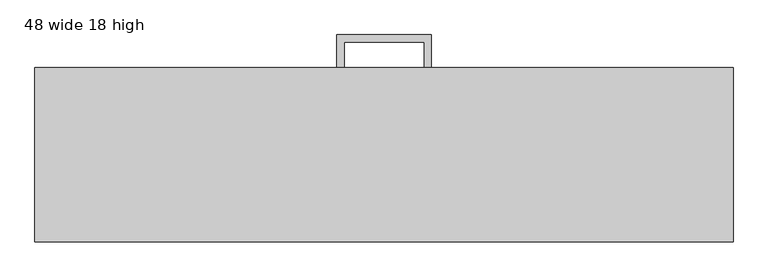
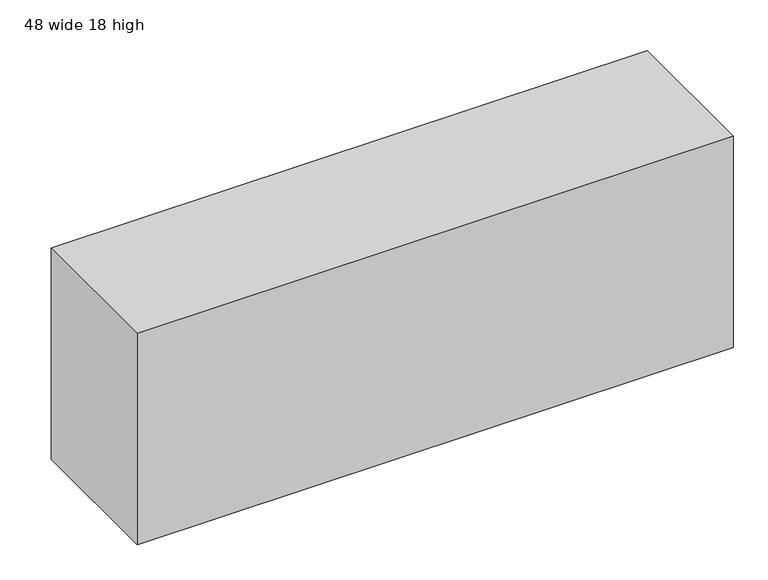
"""IFC4 building model written with IfcOpenShell, lengths in millimetres: furniture geometry, Binder Bin : 48 wide 18 high."""

import ifcopenshell
import ifcopenshell.guid

model = None  # the IFC model being written
_history = None  # IfcOwnerHistory: only IFC2X3 demands one
_inside = {}  # id of a spatial element -> (the spatial element, [elements in it])
_under = {}  # id of a project, library or spatial element -> (it, [spatial elements below it])
_declared = {}  # id of a project -> (the project, [libraries it declares])
_typed = {}  # id of a type object -> (the type object, [elements of that type])
_made_of = {}  # id of a material, layer set ... -> (it, [elements and type objects made of it])


def new_model(schema):
    """Start an empty IFC model of exactly this schema.

    Asked for "IFC4X3", IfcOpenShell would pick the latest addendum, in which some entities
    have other attributes; the version numbers below select the first issue.
    IFC2X3 requires an IfcOwnerHistory on every rooted entity: one is made here for all.
    """
    global model, _history
    if schema == "IFC4X3":
        model = ifcopenshell.file(schema_version=(4, 3, 0, 0))
    else:
        model = ifcopenshell.file(schema=schema)
    _inside.clear()
    _under.clear()
    _declared.clear()
    _typed.clear()
    _made_of.clear()
    _history = None
    if model.schema == "IFC2X3":
        org = make("IfcOrganization", Name="unknown")
        user = make(
            "IfcPersonAndOrganization",
            ThePerson=make("IfcPerson", FamilyName="unknown"),
            TheOrganization=org,
        )
        app = make(
            "IfcApplication",
            ApplicationDeveloper=org,
            Version="unknown",
            ApplicationFullName="unknown",
            ApplicationIdentifier="unknown",
        )
        _history = make(
            "IfcOwnerHistory",
            OwningUser=user,
            OwningApplication=app,
            ChangeAction="ADDED",
            CreationDate=0,
        )
    return model


def make(cls, **values):
    """One entity of the class cls with the attributes given. An attribute that is None is left unset."""
    return model.create_entity(
        cls, **{name: value for name, value in values.items() if value is not None}
    )


def rooted(cls, **values):
    """An entity with a GlobalId (a new one), such as an element, a storey or a relation."""
    return make(cls, GlobalId=ifcopenshell.guid.new(), OwnerHistory=_history, **values)


def si_unit(unit_type, name, prefix=None):
    """IfcSIUnit, for example si_unit("LENGTHUNIT", "METRE", prefix="MILLI")."""
    return make("IfcSIUnit", UnitType=unit_type, Prefix=prefix, Name=name)


def assignment(units):
    """IfcUnitAssignment: the units of a project."""
    return None if units is None else make("IfcUnitAssignment", Units=units)


def point(xyz):
    """IfcCartesianPoint."""
    return None if xyz is None else make("IfcCartesianPoint", Coordinates=xyz)


def direction(xyz):
    """IfcDirection."""
    return None if xyz is None else make("IfcDirection", DirectionRatios=xyz)


def frame(location, z_axis=None, x_axis=None):
    """IfcAxis2Placement3D, a coordinate frame: its origin and axes. An axis left out is left unset."""
    return make(
        "IfcAxis2Placement3D",
        Location=point(location),
        Axis=direction(z_axis),
        RefDirection=direction(x_axis),
    )


def origin():
    """The frame at (0, 0, 0) with its axes left unset."""
    return frame((0.0, 0.0, 0.0))


def place(relative_to, where):
    """IfcLocalPlacement: puts the frame where relative to a parent placement (None: the world)."""
    return make(
        "IfcLocalPlacement", PlacementRelTo=relative_to, RelativePlacement=where
    )


def context(
    kind, dimensions, precision=None, world=None, true_north=None, identifier=None
):
    """IfcGeometricRepresentationContext, for example the 3D "Model" context."""
    return make(
        "IfcGeometricRepresentationContext",
        ContextIdentifier=identifier,
        ContextType=kind,
        CoordinateSpaceDimension=dimensions,
        Precision=precision,
        WorldCoordinateSystem=world,
        TrueNorth=true_north,
    )


def project(units=None, contexts=None):
    """IfcProject with its units and contexts."""
    return rooted(
        "IfcProject",
        Name="project",
        RepresentationContexts=contexts,
        UnitsInContext=assignment(units),
    )


def spatial(cls, under=None, at=None, **own):
    """A site, building, storey or space (cls), placed at a placement, below another one or the project."""
    s = rooted(cls, ObjectPlacement=at, **own)
    if under is not None:
        _under.setdefault(under.id(), (under, []))[1].append(s)
    return s


def polyline(points):
    """IfcPolyline through the points."""
    return make("IfcPolyline", Points=[point(p) for p in points])


def outline(outer, holes=None, kind="AREA"):
    """IfcArbitraryClosedProfileDef: a profile drawn as a closed curve; with holes, ...WithVoids."""
    if holes is None:
        return make("IfcArbitraryClosedProfileDef", ProfileType=kind, OuterCurve=outer)
    return make(
        "IfcArbitraryProfileDefWithVoids",
        ProfileType=kind,
        OuterCurve=outer,
        InnerCurves=holes,
    )


def extrude(swept, where, along, depth):
    """IfcExtrudedAreaSolid: the profile swept, set in the frame where, extruded along a direction by depth."""
    return make(
        "IfcExtrudedAreaSolid",
        SweptArea=swept,
        Position=where,
        ExtrudedDirection=direction(along),
        Depth=depth,
    )


def shape(context_of_items, identifier, shape_type, items):
    """IfcShapeRepresentation: the items that make up one representation, for example the "Body"."""
    return make(
        "IfcShapeRepresentation",
        ContextOfItems=context_of_items,
        RepresentationIdentifier=identifier,
        RepresentationType=shape_type,
        Items=items,
    )


def source(mapping_origin, context_of_items, identifier, shape_type, items):
    """IfcRepresentationMap: a shape defined once, which mapped items show again and again."""
    return make(
        "IfcRepresentationMap",
        MappingOrigin=mapping_origin,
        MappedRepresentation=shape(context_of_items, identifier, shape_type, items),
    )


def transform(
    local_origin,
    x_axis=None,
    y_axis=None,
    z_axis=None,
    scale=None,
    scale2=None,
    scale3=None,
    uniform=True,
):
    """IfcCartesianTransformationOperator3D, or its non-uniform kind. x_axis, y_axis, z_axis: its Axis1, 2, 3."""
    if uniform:
        return make(
            "IfcCartesianTransformationOperator3D",
            Axis1=direction(x_axis),
            Axis2=direction(y_axis),
            LocalOrigin=point(local_origin),
            Scale=scale,
            Axis3=direction(z_axis),
        )
    return make(
        "IfcCartesianTransformationOperator3DnonUniform",
        Axis1=direction(x_axis),
        Axis2=direction(y_axis),
        LocalOrigin=point(local_origin),
        Scale=scale,
        Axis3=direction(z_axis),
        Scale2=scale2,
        Scale3=scale3,
    )


def mapped(mapping_source, mapping_target):
    """IfcMappedItem: shows the shape of a source again, moved by a transform."""
    return make(
        "IfcMappedItem", MappingSource=mapping_source, MappingTarget=mapping_target
    )


def made_of(thing, what):
    """Note that an element or type object is made of a material, layer set ...; save() writes the relation."""
    if what is not None:
        _made_of.setdefault(what.id(), (what, []))[1].append(thing)
    return thing


def element(
    cls,
    number,
    at=None,
    inside=None,
    cuts=None,
    type_object=None,
    material=None,
    context=None,
    identifier="Body",
    shape_type=None,
    held_by="IfcProductDefinitionShape",
    body=None,
    shapes=None,
    **own,
):
    """One element of the class cls, such as IfcWall. Its Tag is "e" and its number.

    at: its placement. inside: the storey or other place that contains it. cuts: it is an
    opening in that element (IfcRelVoidsElement). A single representation is given by context,
    identifier, shape_type and body (its items); several are given by shapes. held_by: the class
    of the entity that holds the representations. save() writes the other relations.
    """
    e = rooted(cls, Tag="e%d" % number, ObjectPlacement=at, **own)
    if body is not None:
        shapes = [shape(context, identifier, shape_type, body)]
    if shapes is not None:
        e.Representation = make(held_by, Representations=shapes)
    if inside is not None:
        _inside.setdefault(inside.id(), (inside, []))[1].append(e)
    if cuts is not None:
        rooted(
            "IfcRelVoidsElement", RelatingBuildingElement=cuts, RelatedOpeningElement=e
        )
    if type_object is not None:
        _typed.setdefault(type_object.id(), (type_object, []))[1].append(e)
    return made_of(e, material)


def aggregate(whole, parts):
    """IfcRelAggregates: a whole, such as a stair, and the parts it consists of."""
    return rooted("IfcRelAggregates", RelatingObject=whole, RelatedObjects=parts)


def save(model, path):
    """Write the relations noted so far, then the file.

    IfcRelAggregates (storeys below a building ...), IfcRelContainedInSpatialStructure (elements
    in a storey), IfcRelDefinesByType, IfcRelAssociatesMaterial and IfcRelDeclares: one each for
    every whole, place, type object, material and project.
    """
    for whole, parts in _under.values():
        aggregate(whole, parts)
    for where, things in _inside.values():
        rooted(
            "IfcRelContainedInSpatialStructure",
            RelatedElements=things,
            RelatingStructure=where,
        )
    for kind, things in _typed.values():
        rooted("IfcRelDefinesByType", RelatedObjects=things, RelatingType=kind)
    for what, things in _made_of.values():
        rooted("IfcRelAssociatesMaterial", RelatedObjects=things, RelatingMaterial=what)
    for by, libraries in _declared.values():
        rooted("IfcRelDeclares", RelatingContext=by, RelatedDefinitions=libraries)
    model.write(path)


def furniture_48_wide_18_high_2f3f987a(model_context):
    return source(origin(), model_context, "Body", "SweptSolid", [
        extrude(outline(polyline([(-69.85, 381.0), (-82.55, 381.0), (-82.55, 438.15), (82.55, 438.15), (82.55, 381.0), (69.85, 381.0), (69.85, 425.45), (-69.85, 425.45), (-69.85, 381.0)])), frame((0.0, 0.0, 1568.45), z_axis=(0.0, 0.0, 1.0), x_axis=(1.0, 0.0, 0.0)), (0.0, 0.0, 1.0), 12.7),
        extrude(outline(polyline([(609.6, 76.2), (-609.6, 76.2), (-609.6, 381.0), (609.6, 381.0), (609.6, 76.2)])), frame((0.0, 0.0, 1524.0), z_axis=(0.0, 0.0, 1.0), x_axis=(1.0, 0.0, 0.0)), (0.0, 0.0, 1.0), 457.2),
    ])


if __name__ == "__main__":
    model = new_model("IFC4")
    model_context = context("Model", 3, world=origin())
    ifc_project = project(units=[si_unit("LENGTHUNIT", "METRE", prefix="MILLI")], contexts=[model_context])
    site = spatial("IfcSite", under=ifc_project)
    building = spatial("IfcBuilding", under=site)
    placement = place(None, origin())
    furniture_48_wide_18_high_shape = furniture_48_wide_18_high_2f3f987a(model_context)
    element("IfcFurniture", 1, ObjectType="Binder Bin : 48 wide 18 high", at=placement, inside=building, context=model_context, shape_type="MappedRepresentation", body=[
        mapped(furniture_48_wide_18_high_shape, transform((0.0, 0.0, 0.0), x_axis=(1.0, 0.0, 0.0), y_axis=(0.0, 1.0, 0.0), z_axis=(0.0, 0.0, 1.0))),
    ])
    save(model, "model.ifc")

# Revit data of these elements
# Type "Binder Bin : 48 wide 18 high"
#   Width = 4' - 0"
#   Mounting Height [instance default] = 4' - 6"
#   Height = 1' - 6"
#   Default Elevation = 0
# Element 1 (IfcFurniture, "Binder Bin : 48 wide 18 high")
#   Mounting Height = 5' - 0"
